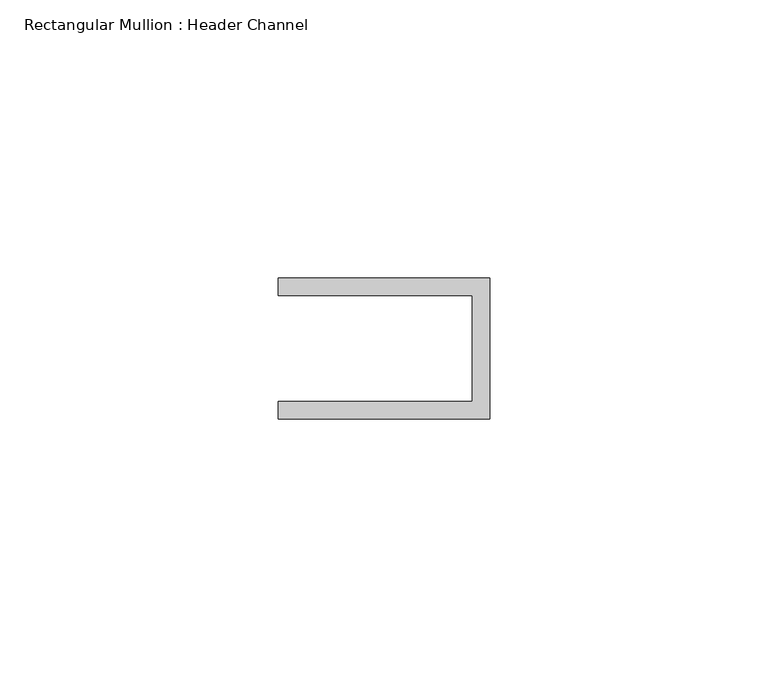
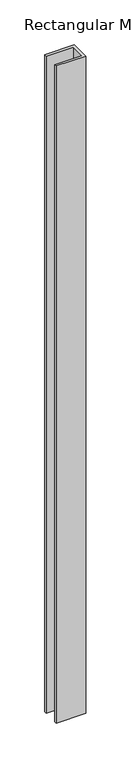
"""IFC4 building model written with IfcOpenShell, lengths in millimetres: member geometry, Rectangular Mullion : Header Channel."""

from ifc_helpers import new_model, si_unit, frame, origin, place, context, project, spatial, polyline, outline, extrude, source, transform, mapped, element, save


def rectangular_mullion_header_channel_d48953c9(model_context):
    return source(origin(), model_context, "Body", "SweptSolid", [
        extrude(outline(polyline([(0.0, -12.7), (-38.1, -12.7), (-38.1, -9.525), (-3.175, -9.525), (-3.175, 9.525), (-38.1, 9.525), (-38.1, 12.7), (0.0, 12.7), (0.0, -12.7)])), frame((0.0, 0.0, -894.3201523), z_axis=(0.0, 0.0, 1.0), x_axis=(1.0, 0.0, 0.0)), (0.0, 0.0, 1.0), 894.3201523),
    ])


if __name__ == "__main__":
    model = new_model("IFC4")
    model_context = context("Model", 3, world=origin())
    ifc_project = project(units=[si_unit("LENGTHUNIT", "METRE", prefix="MILLI")], contexts=[model_context])
    site = spatial("IfcSite", under=ifc_project)
    building = spatial("IfcBuilding", under=site)
    placement = place(None, origin())
    rectangular_mullion_header_channel_shape = rectangular_mullion_header_channel_d48953c9(model_context)
    element("IfcMember", 1, ObjectType="Rectangular Mullion : Header Channel", at=placement, inside=building, context=model_context, shape_type="MappedRepresentation", body=[
        mapped(rectangular_mullion_header_channel_shape, transform((0.0, 0.0, 0.0), x_axis=(1.0, 0.0, 0.0), y_axis=(0.0, 1.0, 0.0), z_axis=(0.0, 0.0, 1.0))),
    ])
    save(model, "model.ifc")

# Revit data of these elements
# Type "Rectangular Mullion : Header Channel"
#   built-in parameter 1007322 = 0.0833333 (stored number, unit not read)
#   built-in parameter 1007321 = -0.03125 (stored number, unit not read)
#   built-in parameter 1007320 = 0.0416667 (stored number, unit not read)
# Element 1 (IfcMember, "Rectangular Mullion : Header Channel")
#   Materials on its faces: "ALUM"
# Materials
#   "ALUM": class "Generic", colour RGB 157 157 157, transparency 0, Cost = 0
